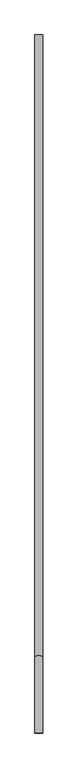
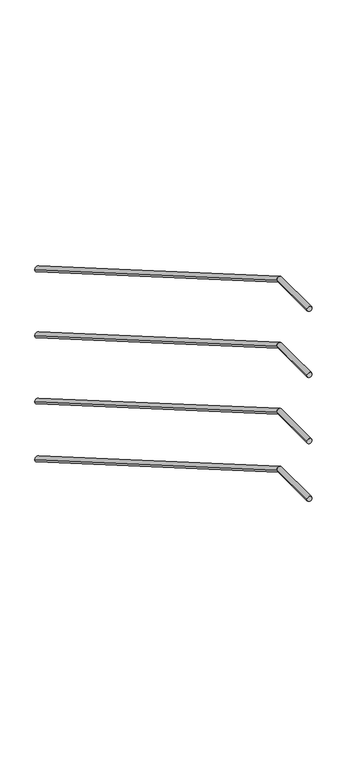
"""IFC4 building model written with IfcOpenShell, lengths in millimetres: railing geometry."""

import ifcopenshell
import ifcopenshell.guid

model = None  # the IFC model being written
_history = None  # IfcOwnerHistory: only IFC2X3 demands one
_inside = {}  # id of a spatial element -> (the spatial element, [elements in it])
_under = {}  # id of a project, library or spatial element -> (it, [spatial elements below it])
_declared = {}  # id of a project -> (the project, [libraries it declares])
_typed = {}  # id of a type object -> (the type object, [elements of that type])
_made_of = {}  # id of a material, layer set ... -> (it, [elements and type objects made of it])


def new_model(schema):
    """Start an empty IFC model of exactly this schema.

    Asked for "IFC4X3", IfcOpenShell would pick the latest addendum, in which some entities
    have other attributes; the version numbers below select the first issue.
    IFC2X3 requires an IfcOwnerHistory on every rooted entity: one is made here for all.
    """
    global model, _history
    if schema == "IFC4X3":
        model = ifcopenshell.file(schema_version=(4, 3, 0, 0))
    else:
        model = ifcopenshell.file(schema=schema)
    _inside.clear()
    _under.clear()
    _declared.clear()
    _typed.clear()
    _made_of.clear()
    _history = None
    if model.schema == "IFC2X3":
        org = make("IfcOrganization", Name="unknown")
        user = make(
            "IfcPersonAndOrganization",
            ThePerson=make("IfcPerson", FamilyName="unknown"),
            TheOrganization=org,
        )
        app = make(
            "IfcApplication",
            ApplicationDeveloper=org,
            Version="unknown",
            ApplicationFullName="unknown",
            ApplicationIdentifier="unknown",
        )
        _history = make(
            "IfcOwnerHistory",
            OwningUser=user,
            OwningApplication=app,
            ChangeAction="ADDED",
            CreationDate=0,
        )
    return model


def make(cls, **values):
    """One entity of the class cls with the attributes given. An attribute that is None is left unset."""
    return model.create_entity(
        cls, **{name: value for name, value in values.items() if value is not None}
    )


def rooted(cls, **values):
    """An entity with a GlobalId (a new one), such as an element, a storey or a relation."""
    return make(cls, GlobalId=ifcopenshell.guid.new(), OwnerHistory=_history, **values)


def si_unit(unit_type, name, prefix=None):
    """IfcSIUnit, for example si_unit("LENGTHUNIT", "METRE", prefix="MILLI")."""
    return make("IfcSIUnit", UnitType=unit_type, Prefix=prefix, Name=name)


def assignment(units):
    """IfcUnitAssignment: the units of a project."""
    return None if units is None else make("IfcUnitAssignment", Units=units)


def point(xyz):
    """IfcCartesianPoint."""
    return None if xyz is None else make("IfcCartesianPoint", Coordinates=xyz)


def direction(xyz):
    """IfcDirection."""
    return None if xyz is None else make("IfcDirection", DirectionRatios=xyz)


def frame(location, z_axis=None, x_axis=None):
    """IfcAxis2Placement3D, a coordinate frame: its origin and axes. An axis left out is left unset."""
    return make(
        "IfcAxis2Placement3D",
        Location=point(location),
        Axis=direction(z_axis),
        RefDirection=direction(x_axis),
    )


def origin():
    """The frame at (0, 0, 0) with its axes left unset."""
    return frame((0.0, 0.0, 0.0))


def place(relative_to, where):
    """IfcLocalPlacement: puts the frame where relative to a parent placement (None: the world)."""
    return make(
        "IfcLocalPlacement", PlacementRelTo=relative_to, RelativePlacement=where
    )


def context(
    kind, dimensions, precision=None, world=None, true_north=None, identifier=None
):
    """IfcGeometricRepresentationContext, for example the 3D "Model" context."""
    return make(
        "IfcGeometricRepresentationContext",
        ContextIdentifier=identifier,
        ContextType=kind,
        CoordinateSpaceDimension=dimensions,
        Precision=precision,
        WorldCoordinateSystem=world,
        TrueNorth=true_north,
    )


def project(units=None, contexts=None):
    """IfcProject with its units and contexts."""
    return rooted(
        "IfcProject",
        Name="project",
        RepresentationContexts=contexts,
        UnitsInContext=assignment(units),
    )


def spatial(cls, under=None, at=None, **own):
    """A site, building, storey or space (cls), placed at a placement, below another one or the project."""
    s = rooted(cls, ObjectPlacement=at, **own)
    if under is not None:
        _under.setdefault(under.id(), (under, []))[1].append(s)
    return s


def circle_curve(where, radius):
    """IfcCircle in the frame where."""
    return make("IfcCircle", Position=where, Radius=radius)


def ellipse_curve(where, semi_axis1, semi_axis2):
    """IfcEllipse in the frame where."""
    return make(
        "IfcEllipse", Position=where, SemiAxis1=semi_axis1, SemiAxis2=semi_axis2
    )


def shape(context_of_items, identifier, shape_type, items):
    """IfcShapeRepresentation: the items that make up one representation, for example the "Body"."""
    return make(
        "IfcShapeRepresentation",
        ContextOfItems=context_of_items,
        RepresentationIdentifier=identifier,
        RepresentationType=shape_type,
        Items=items,
    )


def source(mapping_origin, context_of_items, identifier, shape_type, items):
    """IfcRepresentationMap: a shape defined once, which mapped items show again and again."""
    return make(
        "IfcRepresentationMap",
        MappingOrigin=mapping_origin,
        MappedRepresentation=shape(context_of_items, identifier, shape_type, items),
    )


def transform(
    local_origin,
    x_axis=None,
    y_axis=None,
    z_axis=None,
    scale=None,
    scale2=None,
    scale3=None,
    uniform=True,
):
    """IfcCartesianTransformationOperator3D, or its non-uniform kind. x_axis, y_axis, z_axis: its Axis1, 2, 3."""
    if uniform:
        return make(
            "IfcCartesianTransformationOperator3D",
            Axis1=direction(x_axis),
            Axis2=direction(y_axis),
            LocalOrigin=point(local_origin),
            Scale=scale,
            Axis3=direction(z_axis),
        )
    return make(
        "IfcCartesianTransformationOperator3DnonUniform",
        Axis1=direction(x_axis),
        Axis2=direction(y_axis),
        LocalOrigin=point(local_origin),
        Scale=scale,
        Axis3=direction(z_axis),
        Scale2=scale2,
        Scale3=scale3,
    )


def mapped(mapping_source, mapping_target):
    """IfcMappedItem: shows the shape of a source again, moved by a transform."""
    return make(
        "IfcMappedItem", MappingSource=mapping_source, MappingTarget=mapping_target
    )


def made_of(thing, what):
    """Note that an element or type object is made of a material, layer set ...; save() writes the relation."""
    if what is not None:
        _made_of.setdefault(what.id(), (what, []))[1].append(thing)
    return thing


def element(
    cls,
    number,
    at=None,
    inside=None,
    cuts=None,
    type_object=None,
    material=None,
    context=None,
    identifier="Body",
    shape_type=None,
    held_by="IfcProductDefinitionShape",
    body=None,
    shapes=None,
    **own,
):
    """One element of the class cls, such as IfcWall. Its Tag is "e" and its number.

    at: its placement. inside: the storey or other place that contains it. cuts: it is an
    opening in that element (IfcRelVoidsElement). A single representation is given by context,
    identifier, shape_type and body (its items); several are given by shapes. held_by: the class
    of the entity that holds the representations. save() writes the other relations.
    """
    e = rooted(cls, Tag="e%d" % number, ObjectPlacement=at, **own)
    if body is not None:
        shapes = [shape(context, identifier, shape_type, body)]
    if shapes is not None:
        e.Representation = make(held_by, Representations=shapes)
    if inside is not None:
        _inside.setdefault(inside.id(), (inside, []))[1].append(e)
    if cuts is not None:
        rooted(
            "IfcRelVoidsElement", RelatingBuildingElement=cuts, RelatedOpeningElement=e
        )
    if type_object is not None:
        _typed.setdefault(type_object.id(), (type_object, []))[1].append(e)
    return made_of(e, material)


def aggregate(whole, parts):
    """IfcRelAggregates: a whole, such as a stair, and the parts it consists of."""
    return rooted("IfcRelAggregates", RelatingObject=whole, RelatedObjects=parts)


def save(model, path):
    """Write the relations noted so far, then the file.

    IfcRelAggregates (storeys below a building ...), IfcRelContainedInSpatialStructure (elements
    in a storey), IfcRelDefinesByType, IfcRelAssociatesMaterial and IfcRelDeclares: one each for
    every whole, place, type object, material and project.
    """
    for whole, parts in _under.values():
        aggregate(whole, parts)
    for where, things in _inside.values():
        rooted(
            "IfcRelContainedInSpatialStructure",
            RelatedElements=things,
            RelatingStructure=where,
        )
    for kind, things in _typed.values():
        rooted("IfcRelDefinesByType", RelatedObjects=things, RelatingType=kind)
    for what, things in _made_of.values():
        rooted("IfcRelAssociatesMaterial", RelatedObjects=things, RelatingMaterial=what)
    for by, libraries in _declared.values():
        rooted("IfcRelDeclares", RelatingContext=by, RelatedDefinitions=libraries)
    model.write(path)


def plane_surface(at):
    """IfcPlane: the flat surface through the origin of the frame at, square to its z axis."""
    return make("IfcPlane", Position=at)


def cylinder_surface(at, radius):
    """IfcCylindricalSurface: all points at the distance radius from the z axis of the frame at."""
    return make("IfcCylindricalSurface", Position=at, Radius=radius)


def advanced_brep(points, edges, surfaces, faces):
    """IfcAdvancedBrep: a solid bounded by faces that lie on surfaces and meet in shared edges.

    An edge is (start, end): straight between two places in points (the first is 0);
    or (start, end, curve); or (start, end, curve, False) where it runs against its curve.
    A face is (place in surfaces, loops), or (place, loops, False) where it looks against
    its surface's normal. A loop lists edges by number (the first is 1), with a minus sign
    where the edge is run from its end to its start. The first loop is the outer one.
    """
    corners = [point(p) for p in points]
    vertices = [make("IfcVertexPoint", VertexGeometry=c) for c in corners]
    made = []
    for start, end, *more in edges:
        made.append(
            make(
                "IfcEdgeCurve",
                EdgeStart=vertices[start],
                EdgeEnd=vertices[end],
                EdgeGeometry=more[0] if more else make("IfcPolyline", Points=[corners[start], corners[end]]),
                SameSense=more[1] if len(more) > 1 else True,
            )
        )
    hull = []
    for where, loops, *sense in faces:
        bounds = []
        for j, loop in enumerate(loops):
            ring = [make("IfcOrientedEdge", EdgeElement=made[abs(k) - 1], Orientation=k > 0) for k in loop]
            bounds.append(
                make(
                    "IfcFaceOuterBound" if j == 0 else "IfcFaceBound",
                    Bound=make("IfcEdgeLoop", EdgeList=ring),
                    Orientation=True,
                )
            )
        hull.append(make("IfcAdvancedFace", Bounds=bounds, FaceSurface=surfaces[where], SameSense=sense[0] if sense else True))
    return make("IfcAdvancedBrep", Outer=make("IfcClosedShell", CfsFaces=hull))


def railing_4dfa4352(model_context):
    return source(origin(), model_context, "Body", "AdvancedBrep", [
        advanced_brep(
        [(-1709.6, 15799.5208589, 5689.6773196), (-1739.6, 15799.5208589, 5689.6773196), (-1709.6, 13395.4833005, 7084.9618634), (-1739.6, 13395.4833005, 7084.9618634), (-1709.6, 13099.5208589, 7084.9618634), (-1739.6, 13099.5208589, 7084.9618634)],
        [
            (0, 1, ellipse_curve(frame((-1724.6, 15799.5208589, 5689.6773196), z_axis=(0.0, 1.0, 0.0), x_axis=(0.0, 0.0, -1.0)), 17.3433672, 15.0)),
            (1, 0, ellipse_curve(frame((-1724.6, 15799.5208589, 5689.6773196), z_axis=(0.0, 1.0, 0.0), x_axis=(0.0, 0.0, -1.0)), 17.3433672, 15.0)),
            (0, 2),
            (2, 3, ellipse_curve(frame((-1724.6, 13395.4833005, 7084.9618634), z_axis=(0.0, 0.9656303515230847, -0.25991926480621574), x_axis=(0.0, -0.25991926480621586, -0.9656303515230849)), 15.5338945, 15.0)),
            (3, 1),
            (3, 2, ellipse_curve(frame((-1724.6, 13395.4833005, 7084.9618634), z_axis=(0.0, 0.9656303515230847, -0.25991926480621574), x_axis=(0.0, -0.25991926480621586, -0.9656303515230849)), 15.5338945, 15.0)),
            (4, 5, circle_curve(frame((-1724.6, 13099.5208589, 7084.9618634), z_axis=(0.0, -1.0, 0.0), x_axis=(-1.0, 0.0, 0.0)), 15.0)),
            (5, 4, circle_curve(frame((-1724.6, 13099.5208589, 7084.9618634), z_axis=(0.0, -1.0, 0.0), x_axis=(-1.0, 0.0, 0.0)), 15.0)),
            (2, 4),
            (5, 3),
        ],
        [
            plane_surface(frame((-1724.6, 15799.5208589, 5707.0206869), z_axis=(0.0, 1.0, 0.0), x_axis=(0.0, 0.0, -1.0))),
            cylinder_surface(frame((-1724.6, 15791.991281, 5694.0474276), z_axis=(0.0, 0.8648839515651926, -0.5019718620848959), x_axis=(-1.0, 0.0, 0.0)), 15.0),
            plane_surface(frame((-1724.6, 13099.5208589, 7099.9618634), z_axis=(0.0, -1.0, 0.0), x_axis=(0.0, 0.0, -1.0))),
            cylinder_surface(frame((-1724.6, 13399.5208589, 7084.9618634), z_axis=(0.0, 1.0, 0.0), x_axis=(-1.0, 0.0, 0.0)), 15.0),
        ],
        [
            (0, [[1, 2]]),
            (1, [[-1, 3, 4, 5]]),
            (1, [[-2, -5, 6, -3]]),
            (2, [[7, 8]]),
            (3, [[-4, 9, -8, 10]]),
            (3, [[-6, -10, -7, -9]]),
        ],
    ),
        advanced_brep(
        [(-1709.6, 15799.5208589, 4889.6773196), (-1739.6, 15799.5208589, 4889.6773196), (-1709.6, 13395.4833005, 6284.9618634), (-1739.6, 13395.4833005, 6284.9618634), (-1709.6, 13099.5208589, 6284.9618634), (-1739.6, 13099.5208589, 6284.9618634)],
        [
            (0, 1, ellipse_curve(frame((-1724.6, 15799.5208589, 4889.6773196), z_axis=(0.0, 1.0, 0.0), x_axis=(0.0, 0.0, -1.0)), 17.3433672, 15.0)),
            (1, 0, ellipse_curve(frame((-1724.6, 15799.5208589, 4889.6773196), z_axis=(0.0, 1.0, 0.0), x_axis=(0.0, 0.0, -1.0)), 17.3433672, 15.0)),
            (0, 2),
            (2, 3, ellipse_curve(frame((-1724.6, 13395.4833005, 6284.9618634), z_axis=(0.0, 0.9656303515230847, -0.25991926480621574), x_axis=(0.0, -0.25991926480621586, -0.9656303515230849)), 15.5338945, 15.0)),
            (3, 1),
            (3, 2, ellipse_curve(frame((-1724.6, 13395.4833005, 6284.9618634), z_axis=(0.0, 0.9656303515230847, -0.25991926480621574), x_axis=(0.0, -0.25991926480621586, -0.9656303515230849)), 15.5338945, 15.0)),
            (4, 5, circle_curve(frame((-1724.6, 13099.5208589, 6284.9618634), z_axis=(0.0, -1.0, 0.0), x_axis=(-1.0, 0.0, 0.0)), 15.0)),
            (5, 4, circle_curve(frame((-1724.6, 13099.5208589, 6284.9618634), z_axis=(0.0, -1.0, 0.0), x_axis=(-1.0, 0.0, 0.0)), 15.0)),
            (2, 4),
            (5, 3),
        ],
        [
            plane_surface(frame((-1724.6, 15799.5208589, 4907.0206869), z_axis=(0.0, 1.0, 0.0), x_axis=(0.0, 0.0, -1.0))),
            cylinder_surface(frame((-1724.6, 15791.991281, 4894.0474276), z_axis=(0.0, 0.8648839515651926, -0.5019718620848959), x_axis=(-1.0, 0.0, 0.0)), 15.0),
            plane_surface(frame((-1724.6, 13099.5208589, 6299.9618634), z_axis=(0.0, -1.0, 0.0), x_axis=(0.0, 0.0, -1.0))),
            cylinder_surface(frame((-1724.6, 13399.5208589, 6284.9618634), z_axis=(0.0, 1.0, 0.0), x_axis=(-1.0, 0.0, 0.0)), 15.0),
        ],
        [
            (0, [[1, 2]]),
            (1, [[-1, 3, 4, 5]]),
            (1, [[-2, -5, 6, -3]]),
            (2, [[7, 8]]),
            (3, [[-4, 9, -8, 10]]),
            (3, [[-6, -10, -7, -9]]),
        ],
    ),
        advanced_brep(
        [(-1709.6, 15799.5208589, 5289.6773196), (-1739.6, 15799.5208589, 5289.6773196), (-1709.6, 13395.4833005, 6684.9618634), (-1739.6, 13395.4833005, 6684.9618634), (-1709.6, 13099.5208589, 6684.9618634), (-1739.6, 13099.5208589, 6684.9618634)],
        [
            (0, 1, ellipse_curve(frame((-1724.6, 15799.5208589, 5289.6773196), z_axis=(0.0, 1.0, 0.0), x_axis=(0.0, 0.0, -1.0)), 17.3433672, 15.0)),
            (1, 0, ellipse_curve(frame((-1724.6, 15799.5208589, 5289.6773196), z_axis=(0.0, 1.0, 0.0), x_axis=(0.0, 0.0, -1.0)), 17.3433672, 15.0)),
            (0, 2),
            (2, 3, ellipse_curve(frame((-1724.6, 13395.4833005, 6684.9618634), z_axis=(0.0, 0.9656303515230847, -0.25991926480621574), x_axis=(0.0, -0.25991926480621586, -0.9656303515230849)), 15.5338945, 15.0)),
            (3, 1),
            (3, 2, ellipse_curve(frame((-1724.6, 13395.4833005, 6684.9618634), z_axis=(0.0, 0.9656303515230847, -0.25991926480621574), x_axis=(0.0, -0.25991926480621586, -0.9656303515230849)), 15.5338945, 15.0)),
            (4, 5, circle_curve(frame((-1724.6, 13099.5208589, 6684.9618634), z_axis=(0.0, -1.0, 0.0), x_axis=(-1.0, 0.0, 0.0)), 15.0)),
            (5, 4, circle_curve(frame((-1724.6, 13099.5208589, 6684.9618634), z_axis=(0.0, -1.0, 0.0), x_axis=(-1.0, 0.0, 0.0)), 15.0)),
            (2, 4),
            (5, 3),
        ],
        [
            plane_surface(frame((-1724.6, 15799.5208589, 5307.0206869), z_axis=(0.0, 1.0, 0.0), x_axis=(0.0, 0.0, -1.0))),
            cylinder_surface(frame((-1724.6, 15791.991281, 5294.0474276), z_axis=(0.0, 0.8648839515651926, -0.5019718620848959), x_axis=(-1.0, 0.0, 0.0)), 15.0),
            plane_surface(frame((-1724.6, 13099.5208589, 6699.9618634), z_axis=(0.0, -1.0, 0.0), x_axis=(0.0, 0.0, -1.0))),
            cylinder_surface(frame((-1724.6, 13399.5208589, 6684.9618634), z_axis=(0.0, 1.0, 0.0), x_axis=(-1.0, 0.0, 0.0)), 15.0),
        ],
        [
            (0, [[1, 2]]),
            (1, [[-1, 3, 4, 5]]),
            (1, [[-2, -5, 6, -3]]),
            (2, [[7, 8]]),
            (3, [[-4, 9, -8, 10]]),
            (3, [[-6, -10, -7, -9]]),
        ],
    ),
        advanced_brep(
        [(-1709.6, 15799.5208589, 4539.6773196), (-1739.6, 15799.5208589, 4539.6773196), (-1709.6, 13395.4833005, 5934.9618634), (-1739.6, 13395.4833005, 5934.9618634), (-1709.6, 13099.5208589, 5934.9618634), (-1739.6, 13099.5208589, 5934.9618634)],
        [
            (0, 1, ellipse_curve(frame((-1724.6, 15799.5208589, 4539.6773196), z_axis=(0.0, 1.0, 0.0), x_axis=(0.0, 0.0, -1.0)), 17.3433672, 15.0)),
            (1, 0, ellipse_curve(frame((-1724.6, 15799.5208589, 4539.6773196), z_axis=(0.0, 1.0, 0.0), x_axis=(0.0, 0.0, -1.0)), 17.3433672, 15.0)),
            (0, 2),
            (2, 3, ellipse_curve(frame((-1724.6, 13395.4833005, 5934.9618634), z_axis=(0.0, 0.9656303515230847, -0.25991926480621574), x_axis=(0.0, -0.25991926480621586, -0.9656303515230849)), 15.5338945, 15.0)),
            (3, 1),
            (3, 2, ellipse_curve(frame((-1724.6, 13395.4833005, 5934.9618634), z_axis=(0.0, 0.9656303515230847, -0.25991926480621574), x_axis=(0.0, -0.25991926480621586, -0.9656303515230849)), 15.5338945, 15.0)),
            (4, 5, circle_curve(frame((-1724.6, 13099.5208589, 5934.9618634), z_axis=(0.0, -1.0, 0.0), x_axis=(-1.0, 0.0, 0.0)), 15.0)),
            (5, 4, circle_curve(frame((-1724.6, 13099.5208589, 5934.9618634), z_axis=(0.0, -1.0, 0.0), x_axis=(-1.0, 0.0, 0.0)), 15.0)),
            (2, 4),
            (5, 3),
        ],
        [
            plane_surface(frame((-1724.6, 15799.5208589, 4557.0206869), z_axis=(0.0, 1.0, 0.0), x_axis=(0.0, 0.0, -1.0))),
            cylinder_surface(frame((-1724.6, 15791.991281, 4544.0474276), z_axis=(0.0, 0.8648839515651926, -0.5019718620848959), x_axis=(-1.0, 0.0, 0.0)), 15.0),
            plane_surface(frame((-1724.6, 13099.5208589, 5949.9618634), z_axis=(0.0, -1.0, 0.0), x_axis=(0.0, 0.0, -1.0))),
            cylinder_surface(frame((-1724.6, 13399.5208589, 5934.9618634), z_axis=(0.0, 1.0, 0.0), x_axis=(-1.0, 0.0, 0.0)), 15.0),
        ],
        [
            (0, [[1, 2]]),
            (1, [[-1, 3, 4, 5]]),
            (1, [[-2, -5, 6, -3]]),
            (2, [[7, 8]]),
            (3, [[-4, 9, -8, 10]]),
            (3, [[-6, -10, -7, -9]]),
        ],
    ),
    ])


if __name__ == "__main__":
    model = new_model("IFC4")
    model_context = context("Model", 3, world=origin())
    ifc_project = project(units=[si_unit("LENGTHUNIT", "METRE", prefix="MILLI")], contexts=[model_context])
    site = spatial("IfcSite", under=ifc_project)
    building = spatial("IfcBuilding", under=site)
    placement = place(None, origin())
    railing_shape = railing_4dfa4352(model_context)
    element("IfcRailing", 1, at=placement, inside=building, context=model_context, shape_type="MappedRepresentation", body=[
        mapped(railing_shape, transform((0.0, 0.0, 0.0), x_axis=(1.0, 0.0, 0.0), y_axis=(0.0, 1.0, 0.0), z_axis=(0.0, 0.0, 1.0))),
    ])
    save(model, "model.ifc")
